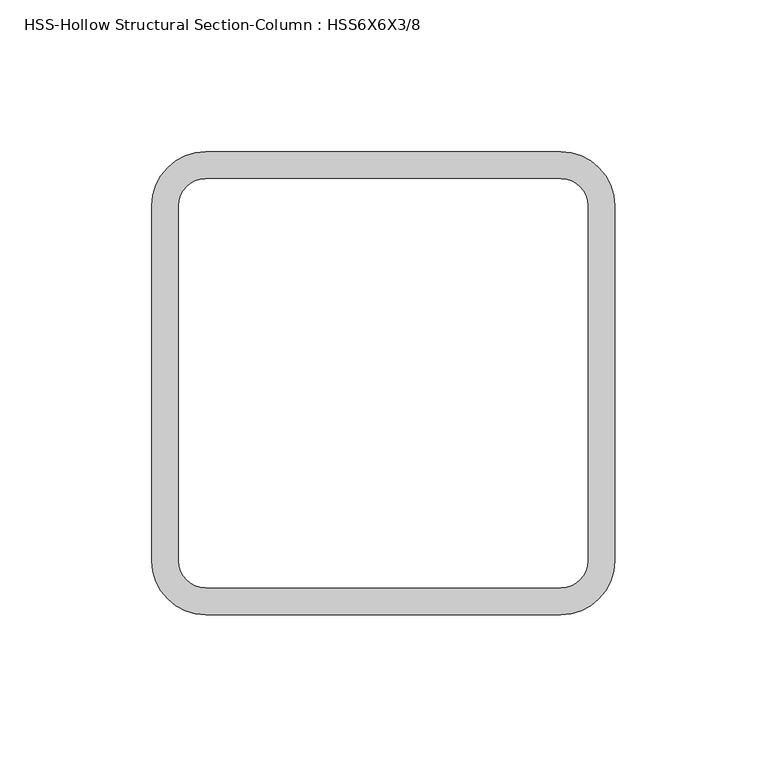
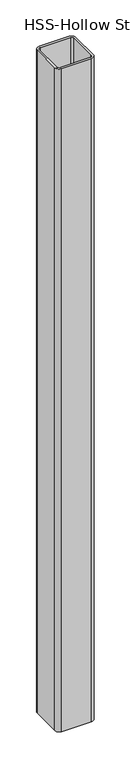
"""IFC4 building model written with IfcOpenShell, lengths in millimetres: column geometry, HSS-Hollow Structural Section-Column : HSS6X6X3/8."""

from ifc_helpers import new_model, si_unit, point, frame, frame_2d, origin, place, context, project, spatial, polyline, circle_curve, trimmed, segment, composite_curve, outline, extrude, source, transform, mapped, element, save


def hss_hollow_structural_section_column_hss6x6x3_8_70018103(model_context):
    return source(origin(), model_context, "Body", "SweptSolid", [
        extrude(outline(composite_curve([segment(trimmed(circle_curve(frame_2d((58.4708, 58.4708)), 17.7292), [point((58.4708, 76.2))], [point((76.2, 58.4708))], False, "CARTESIAN"), True, "CONTINUOUS"), segment(polyline([(76.2, 58.4708), (76.2, -58.4708)]), True, "CONTINUOUS"), segment(trimmed(circle_curve(frame_2d((58.4708, -58.4708)), 17.7292), [point((76.2, -58.4708))], [point((58.4708, -76.2))], False, "CARTESIAN"), True, "CONTINUOUS"), segment(polyline([(58.4708, -76.2), (-58.4708, -76.2)]), True, "CONTINUOUS"), segment(trimmed(circle_curve(frame_2d((-58.4708, -58.4708)), 17.7292), [point((-58.4708, -76.2))], [point((-76.2, -58.4708))], False, "CARTESIAN"), True, "CONTINUOUS"), segment(polyline([(-76.2, -58.4708), (-76.2, 58.4708)]), True, "CONTINUOUS"), segment(trimmed(circle_curve(frame_2d((-58.4708, 58.4708)), 17.7292), [point((-76.2, 58.4708))], [point((-58.4708, 76.2))], False, "CARTESIAN"), True, "CONTINUOUS"), segment(polyline([(-58.4708, 76.2), (58.4708, 76.2)]), True, "CONTINUOUS")], self_intersect=False), holes=[composite_curve([segment(polyline([(58.4708, 67.3354), (-58.4708, 67.3354)]), True, "CONTINUOUS"), segment(trimmed(circle_curve(frame_2d((-58.4708, 58.4708)), 8.8646), [point((-58.4708, 67.3354))], [point((-67.3354, 58.4708))], True, "CARTESIAN"), True, "CONTINUOUS"), segment(polyline([(-67.3354, 58.4708), (-67.3354, -58.4708)]), True, "CONTINUOUS"), segment(trimmed(circle_curve(frame_2d((-58.4708, -58.4708)), 8.8646), [point((-67.3354, -58.4708))], [point((-58.4708, -67.3354))], True, "CARTESIAN"), True, "CONTINUOUS"), segment(polyline([(-58.4708, -67.3354), (58.4708, -67.3354)]), True, "CONTINUOUS"), segment(trimmed(circle_curve(frame_2d((58.4708, -58.4708)), 8.8646), [point((58.4708, -67.3354))], [point((67.3354, -58.4708))], True, "CARTESIAN"), True, "CONTINUOUS"), segment(polyline([(67.3354, -58.4708), (67.3354, 58.4708)]), True, "CONTINUOUS"), segment(trimmed(circle_curve(frame_2d((58.4708, 58.4708)), 8.8646), [point((67.3354, 58.4708))], [point((58.4708, 67.3354))], True, "CARTESIAN"), True, "CONTINUOUS")], self_intersect=False)]), frame((0.0, 0.0, 12566.65), z_axis=(0.0, 0.0, 1.0), x_axis=(1.0, 0.0, 0.0)), (0.0, 0.0, 1.0), 2743.2),
    ])


if __name__ == "__main__":
    model = new_model("IFC4")
    model_context = context("Model", 3, world=origin())
    ifc_project = project(units=[si_unit("LENGTHUNIT", "METRE", prefix="MILLI")], contexts=[model_context])
    site = spatial("IfcSite", under=ifc_project)
    building = spatial("IfcBuilding", under=site)
    placement = place(None, origin())
    hss_hollow_structural_section_column_hss6x6x3_8_shape = hss_hollow_structural_section_column_hss6x6x3_8_70018103(model_context)
    element("IfcColumn", 1, ObjectType="HSS-Hollow Structural Section-Column : HSS6X6X3/8", at=placement, inside=building, context=model_context, shape_type="MappedRepresentation", body=[
        mapped(hss_hollow_structural_section_column_hss6x6x3_8_shape, transform((0.0, 0.0, 0.0), x_axis=(1.0, 0.0, 0.0), y_axis=(0.0, 1.0, 0.0), z_axis=(0.0, 0.0, 1.0))),
    ])
    save(model, "model.ifc")

# Revit data of these elements
# Type "HSS-Hollow Structural Section-Column : HSS6X6X3/8"
#   Assembly Code = "B10"
#   Shape = "Square"
#   W = 27.4
#   Ht = 0' - 6"
#   b = 0' - 6"
#   kr = 0' - 0.698"
#   t = 0' - 0.349"
#   A = 0.0526389 SF
#   Structural Material [instance default] = Steel ASTM A500, Grade B, Rectangular and Square
# Element 1 (IfcColumn, "HSS-Hollow Structural Section-Column : HSS6X6X3/8")
#   Materials on its faces: "Steel ASTM A500, Grade B, Rectangular and Square"
# Materials
#   "Steel ASTM A500, Grade B, Rectangular and Square": class "Metal", colour RGB 199 199 199, transparency 0, Description = "Carbon steel", Cost = 0
